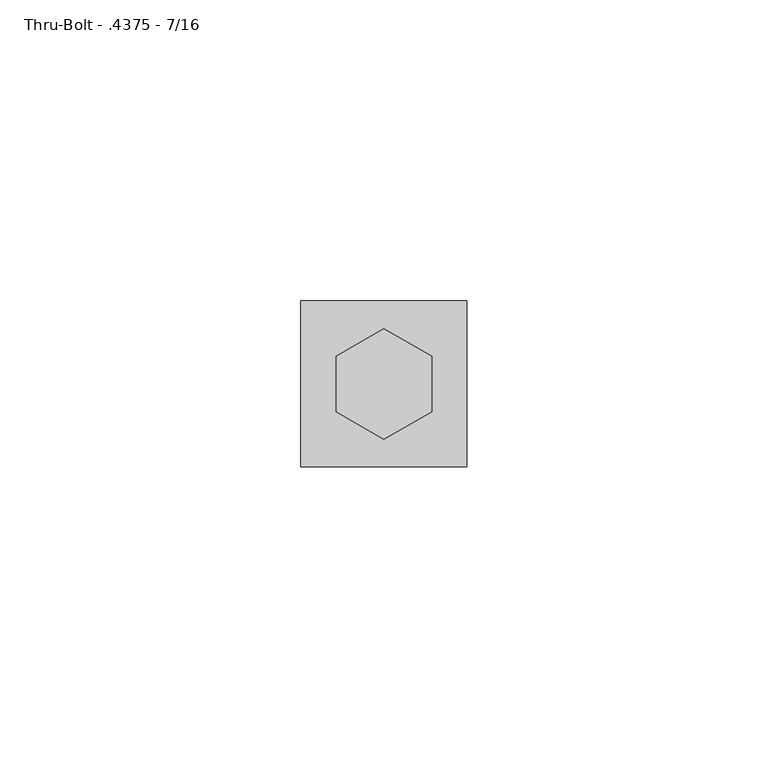
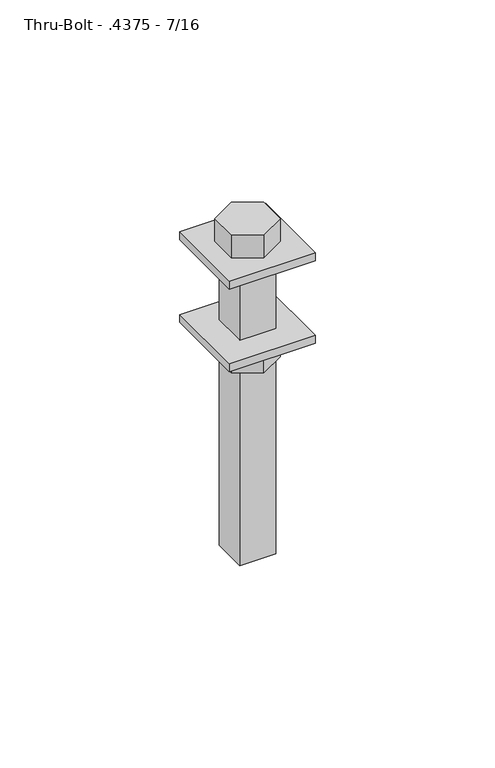
"""IFC4 building model written with IfcOpenShell, lengths in millimetres: fastener geometry, 060523 - W_P_C - Fastenings - Generic - SQUARE : Thru-Bolt - .4375 - 7/16."""

from ifc_helpers import new_model, si_unit, frame, origin, origin_with_axes, place, context, project, spatial, polyline, outline, extrude, source, transform, mapped, element, save


def thru_bolt_4375_7_16_bbfdf3dc(model_context):
    return source(origin(), model_context, "Body", "SweptSolid", [
        extrude(outline(polyline([(-13.7914063, -13.7914063), (-13.7914063, 13.7914062), (13.7914062, 13.7914062), (13.7914062, -13.7914063), (-13.7914063, -13.7914063)])), origin_with_axes(), (0.0, 0.0, 1.0), 2.6789062),
        extrude(outline(polyline([(-13.7914063, -13.7914063), (-13.7914063, 13.7914062), (13.7914062, 13.7914062), (13.7914062, -13.7914063), (-13.7914063, -13.7914063)])), frame((0.0, 0.0, -28.0789063), z_axis=(0.0, 0.0, 1.0), x_axis=(1.0, 0.0, 0.0)), (0.0, 0.0, 1.0), 2.6789062),
        extrude(outline(polyline([(-7.9375, -4.5827178), (-7.9375, 4.5827178), (0.0, 9.1654355), (7.9375, 4.5827178), (7.9375, -4.5827178), (0.0, -9.1654355), (-7.9375, -4.5827178)])), frame((0.0, 0.0, -36.115625), z_axis=(0.0, 0.0, 1.0), x_axis=(1.0, 0.0, 0.0)), (0.0, 0.0, 1.0), 8.0367187),
        extrude(outline(polyline([(-7.9375, 4.5827178), (0.0, 9.1654355), (7.9375, 4.5827178), (7.9375, -4.5827178), (0.0, -9.1654355), (-7.9375, -4.5827178), (-7.9375, 4.5827178)])), frame((0.0, 0.0, 2.6789063), z_axis=(0.0, 0.0, 1.0), x_axis=(1.0, 0.0, 0.0)), (0.0, 0.0, 1.0), 8.0367187),
        extrude(outline(polyline([(-5.7546875, 5.7546875), (5.7546875, 5.7546875), (5.7546875, -5.7546875), (-5.7546875, -5.7546875), (-5.7546875, 5.7546875)])), frame((0.0, 0.0, -101.6), z_axis=(0.0, 0.0, 1.0), x_axis=(1.0, 0.0, 0.0)), (0.0, 0.0, 1.0), 104.2789062),
    ])


if __name__ == "__main__":
    model = new_model("IFC4")
    model_context = context("Model", 3, world=origin())
    ifc_project = project(units=[si_unit("LENGTHUNIT", "METRE", prefix="MILLI")], contexts=[model_context])
    site = spatial("IfcSite", under=ifc_project)
    building = spatial("IfcBuilding", under=site)
    placement = place(None, origin())
    thru_bolt_4375_7_16_shape = thru_bolt_4375_7_16_bbfdf3dc(model_context)
    element("IfcFastener", 1, ObjectType="060523 - W_P_C - Fastenings - Generic - SQUARE : Thru-Bolt - .4375 - 7/16", at=placement, inside=building, context=model_context, shape_type="MappedRepresentation", body=[
        mapped(thru_bolt_4375_7_16_shape, transform((0.0, 0.0, 0.0), x_axis=(1.0, 0.0, 0.0), y_axis=(0.0, 1.0, 0.0), z_axis=(0.0, 0.0, 1.0))),
    ])
    save(model, "model.ifc")

# Revit data of these elements
# Type "060523 - W_P_C - Fastenings - Generic - SQUARE : Thru-Bolt - .4375 - 7/16"
#   Washer_Thickness = 0' - 0 27/256"
#   Washer Radius = 0' - 0 139/256"
#   Washer Offset - Head = 0' - 0 27/256"
#   Washer Offset = 0' - 0 27/256"
#   Thickness_of_Substrate [instance default] = 0' - 1"
#   Side = 0' - 0.36133"
#   Radius = 0' - 0 29/128"
#   Length [instance default] = 0' - 4"
#   Head Size = 0' - 0 5/8"
#   Head Radius = 0' - 0 5/16"
#   Head Height = 0' - 0 81/256"
#   Double Diameter = 0' - 0 29/32"
#   Diameter = 0' - 0 29/64"
#   Default Elevation = 4' - 0"
#   Washer_Nut_Visibility = yes
#   Washer_Head_Visibility = yes
#   Round_Head_Visibility = no
#   Point Visibility = no
#   Nut_Visibility = yes
#   Hex_Head_Visiblilty = yes
#   Washer Material = none
#   Bolt Material (Size) = AT SILL - FASTENER AT 24" O.C.
# Element 1 (IfcFastener, "060523 - W_P_C - Fastenings - Generic - SQUARE : Thru-Bolt - .4375 - 7/16")
#   Materials on its faces: "AT SILL - FASTENER AT 24\" O.C."
# Materials
#   "AT SILL - FASTENER AT 24\" O.C.": class "Generic", colour RGB 120 120 120, transparency 0, Cost = 0
